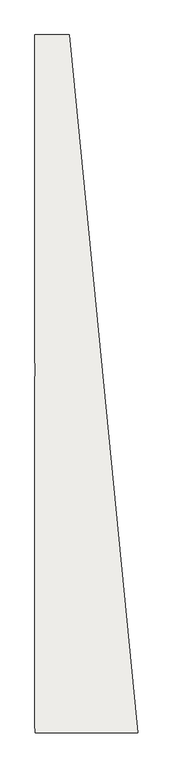
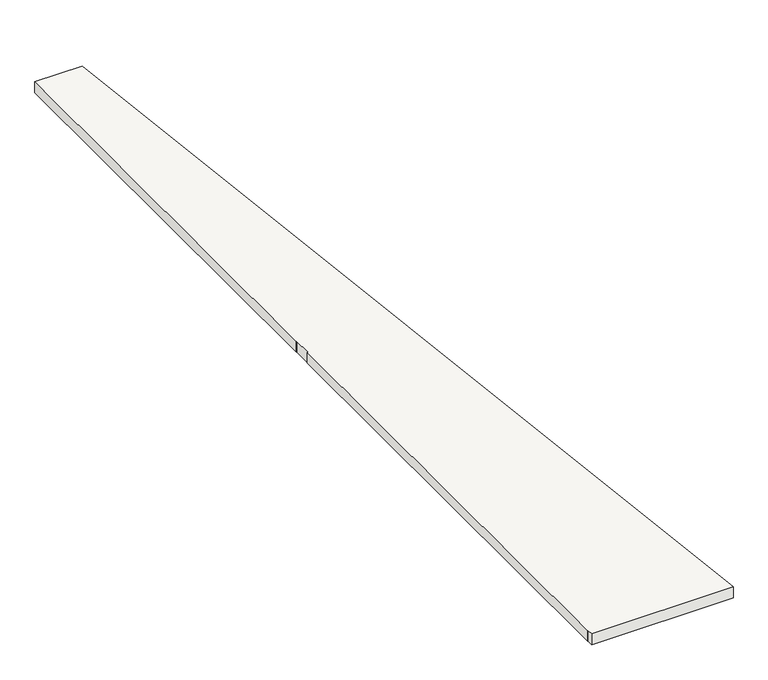
"""IFC4 building model written with IfcOpenShell, lengths in millimetres: slab geometry, Pano 2 (12 cm)."""

from ifc_helpers import new_model, si_unit, origin, origin_with_axes, place, context, project, spatial, polyline, outline, extrude, source, transform, mapped, element, save


def slab_a837895f(model_context):
    return source(origin(), model_context, "Body", "SweptSolid", [
        extrude(outline(polyline([(9395.0, 5550.0), (9395.0, 10350.61224), (9899.44978, 10350.61224), (10900.4902, 140.0), (9400.0, 140.0), (9400.0, 200.0), (9395.0, 200.0), (9395.0, 5350.0), (9400.0, 5350.0), (9400.0, 5550.0), (9395.0, 5550.0)])), origin_with_axes(), (0.0, 0.0, 1.0), 120.0),
    ])


if __name__ == "__main__":
    model = new_model("IFC4")
    model_context = context("Model", 3, world=origin())
    ifc_project = project(units=[si_unit("LENGTHUNIT", "METRE", prefix="MILLI")], contexts=[model_context])
    site = spatial("IfcSite", under=ifc_project)
    building = spatial("IfcBuilding", under=site)
    placement = place(None, origin())
    slab_shape = slab_a837895f(model_context)
    element("IfcSlab", 1, ObjectType="Pano 2 (12 cm)", at=placement, inside=building, context=model_context, shape_type="MappedRepresentation", body=[
        mapped(slab_shape, transform((0.0, 0.0, 0.0), x_axis=(1.0, 0.0, 0.0), y_axis=(0.0, 1.0, 0.0), z_axis=(0.0, 0.0, 1.0))),
    ])
    save(model, "model.ifc")

# Revit data of these elements
# Element 1 (IfcSlab, "Pano 2 (12 cm)")
#   Materials on its faces: "RGB 168-169-158"
# Materials
#   "RGB 168-169-158": class "Não atribuído", colour RGB 168 169 158, transparency 0
